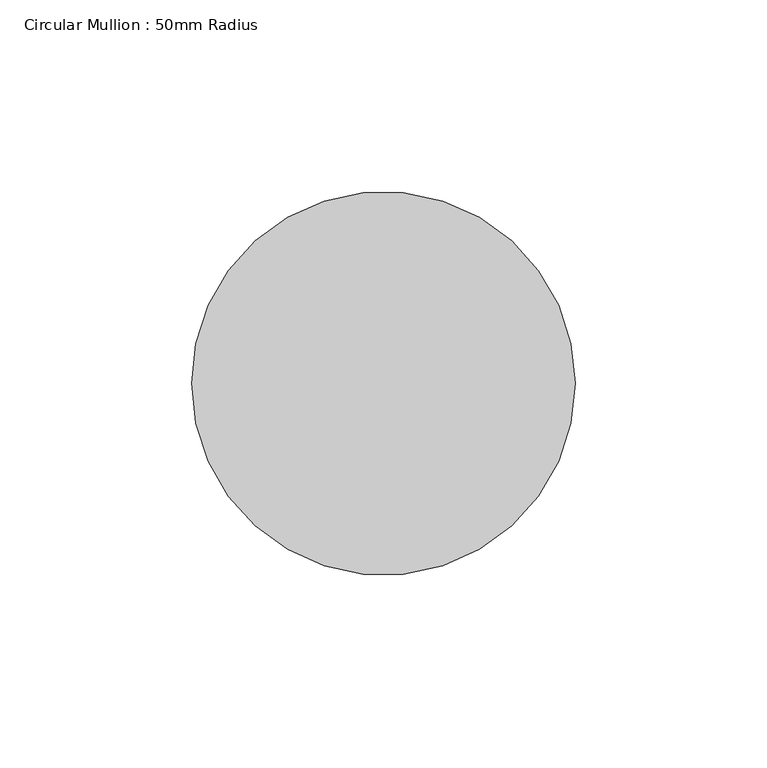
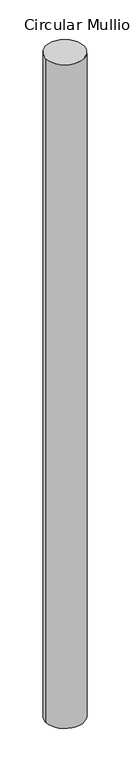
"""IFC4 building model written with IfcOpenShell, lengths in millimetres: member geometry, Circular Mullion : 50mm Radius."""

from ifc_helpers import new_model, si_unit, point, frame, origin, origin_2d, place, context, project, spatial, circle_curve, trimmed, segment, composite_curve, outline, extrude, source, transform, mapped, element, save


def circular_mullion_50mm_radius_ff4871fb(model_context):
    return source(origin(), model_context, "Body", "SweptSolid", [
        extrude(outline(composite_curve([segment(trimmed(circle_curve(origin_2d(), 50.0), [point((50.0, 0.0))], [point((-50.0, 0.0))], False, "CARTESIAN"), True, "CONTINUOUS"), segment(trimmed(circle_curve(origin_2d(), 50.0), [point((-50.0, 0.0))], [point((50.0, 0.0))], False, "CARTESIAN"), True, "CONTINUOUS")], self_intersect=False)), frame((0.0, 0.0, -1836.9242046), z_axis=(0.0, 0.0, 1.0), x_axis=(1.0, 0.0, 0.0)), (0.0, 0.0, 1.0), 1836.9242046),
    ])


if __name__ == "__main__":
    model = new_model("IFC4")
    model_context = context("Model", 3, world=origin())
    ifc_project = project(units=[si_unit("LENGTHUNIT", "METRE", prefix="MILLI")], contexts=[model_context])
    site = spatial("IfcSite", under=ifc_project)
    building = spatial("IfcBuilding", under=site)
    placement = place(None, origin())
    circular_mullion_50mm_radius_shape = circular_mullion_50mm_radius_ff4871fb(model_context)
    element("IfcMember", 1, ObjectType="Circular Mullion : 50mm Radius", at=placement, inside=building, context=model_context, shape_type="MappedRepresentation", body=[
        mapped(circular_mullion_50mm_radius_shape, transform((0.0, 0.0, 0.0), x_axis=(1.0, 0.0, 0.0), y_axis=(0.0, 1.0, 0.0), z_axis=(0.0, 0.0, 1.0))),
    ])
    save(model, "model.ifc")

# Revit data of these elements
# Type "Circular Mullion : 50mm Radius"
#   built-in parameter 1007350 = 0.164042 (stored number, unit not read)
# Element 1 (IfcMember, "Circular Mullion : 50mm Radius")
#   Materials on its faces: "Aluminium"
# Materials
#   "Aluminium": class "Metal", colour RGB 247 247 247, transparency 0, Description = "Aluminium 6061", Cost = 0
